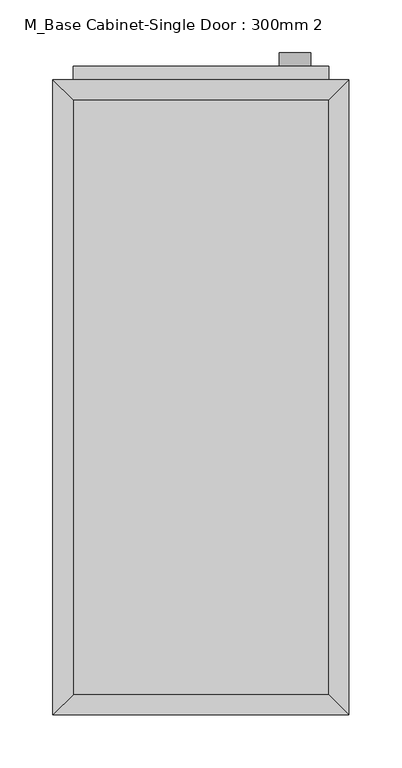
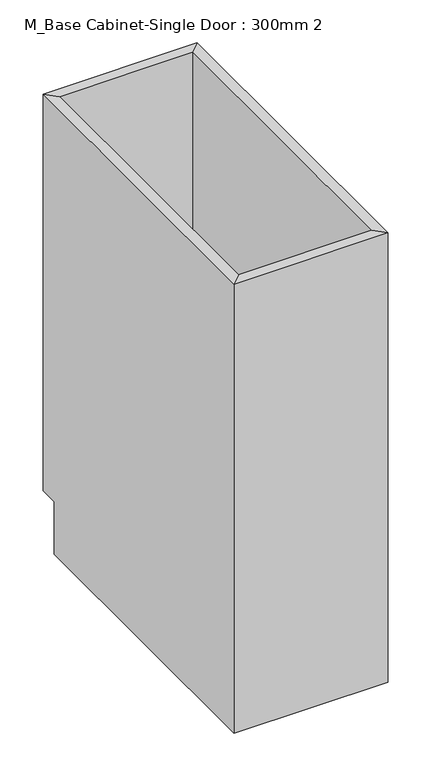
"""IFC4 building model written with IfcOpenShell, lengths in millimetres: furniture geometry, M_Base Cabinet-Single Door : 300mm 2."""

from ifc_helpers import new_model, si_unit, point, frame, frame_2d, origin, place, context, project, spatial, polyline, circle_curve, trimmed, segment, composite_curve, outline, extrude, faceted_brep, source, transform, mapped, element, save


def m_base_cabinet_single_door_300mm_2_2f133583(model_context):
    return source(origin(), model_context, "Body", "SolidModel", [
        faceted_brep([(139.3877049, 580.95, 860.0), (-101.9122951, 580.95, 860.0), (-101.9122951, 580.95, 100.0), (139.3877049, 580.95, 100.0), (158.4377049, 600.0, 860.0), (-120.9622951, 600.0, 860.0), (158.4377049, 600.0, 100.0), (-120.9622951, 600.0, 100.0), (-101.9122951, 19.05, 860.0), (-101.9122951, 19.05, 100.0), (-101.9122951, 565.0, 100.0), (-120.9622951, 0.0, 860.0), (-120.9622951, 565.0, 100.0), (-120.9622951, 565.0, 0.0), (-120.9622951, 0.0, 0.0), (139.3877049, 19.05, 860.0), (139.3877049, 19.05, 100.0), (158.4377049, 0.0, 860.0), (158.4377049, 0.0, 0.0), (139.3877049, 565.0, 100.0), (158.4377049, 565.0, 0.0), (158.4377049, 565.0, 100.0)], [[[0, 1, 2, 3]], [[0, 4, 5, 1]], [[4, 6, 7, 5]], [[2, 7, 6, 3]], [[1, 8, 9, 10, 2]], [[5, 11, 8, 1]], [[7, 12, 13, 14, 11, 5]], [[2, 10, 12, 7]], [[8, 15, 16, 9]], [[11, 17, 15, 8]], [[14, 18, 17, 11]], [[3, 19, 16, 15, 0]], [[0, 15, 17, 4]], [[4, 17, 18, 20, 21, 6]], [[6, 21, 19, 3]], [[10, 9, 16, 19]], [[18, 14, 13, 20]], [[13, 12, 10, 19, 21, 20]]]),
        extrude(outline(composite_curve([segment(trimmed(circle_curve(frame_2d((752.05, 107.6377049)), 15.0), [point((752.05, 92.6377049))], [point((752.05, 122.6377049))], False, "CARTESIAN"), True, "CONTINUOUS"), segment(trimmed(circle_curve(frame_2d((752.05, 107.6377049)), 15.0), [point((752.05, 122.6377049))], [point((752.05, 92.6377049))], False, "CARTESIAN"), True, "CONTINUOUS")], self_intersect=False)), frame((0.0, 612.7, 0.0), z_axis=(0.0, 1.0, 0.0), x_axis=(0.0, 0.0, 1.0)), (0.0, 0.0, 1.0), 12.7),
        extrude(outline(polyline([(139.3877049, 612.7), (139.3877049, 600.0), (-101.9122951, 600.0), (-101.9122951, 612.7), (139.3877049, 612.7)])), frame((0.0, 0.0, 119.05), z_axis=(0.0, 0.0, 1.0), x_axis=(1.0, 0.0, 0.0)), (0.0, 0.0, 1.0), 721.9),
        extrude(outline(polyline([(139.3877049, 19.05), (-101.9122951, 19.05), (-101.9122951, 580.95), (139.3877049, 580.95), (139.3877049, 19.05)])), frame((0.0, 0.0, 100.0), z_axis=(0.0, 0.0, 1.0), x_axis=(1.0, 0.0, 0.0)), (0.0, 0.0, 1.0), 19.05),
    ])


if __name__ == "__main__":
    model = new_model("IFC4")
    model_context = context("Model", 3, world=origin())
    ifc_project = project(units=[si_unit("LENGTHUNIT", "METRE", prefix="MILLI")], contexts=[model_context])
    site = spatial("IfcSite", under=ifc_project)
    building = spatial("IfcBuilding", under=site)
    placement = place(None, origin())
    m_base_cabinet_single_door_300mm_2_shape = m_base_cabinet_single_door_300mm_2_2f133583(model_context)
    element("IfcFurniture", 1, ObjectType="M_Base Cabinet-Single Door : 300mm 2", at=placement, inside=building, context=model_context, shape_type="MappedRepresentation", body=[
        mapped(m_base_cabinet_single_door_300mm_2_shape, transform((0.0, 0.0, 0.0), x_axis=(1.0, 0.0, 0.0), y_axis=(0.0, 1.0, 0.0), z_axis=(0.0, 0.0, 1.0))),
    ])
    save(model, "model.ifc")

# Revit data of these elements
# Type "M_Base Cabinet-Single Door : 300mm 2"
#   Depth = 1' - 11.62205"
#   Height = 2' - 9.85827"
#   Plinth Depth = 0' - 1.37795"
#   Plinth Height = 0' - 3.93701"
#   Width = 0' - 11"
#   Cabinet Material = Base cabinet 2120100 Aspekt - 83012120100 - White
#   Drawer Material = Base cabinet 2120100 Aspekt - 83012120100 - White
#   Handle Material = Cabinets - Handles
#   Default Elevation = 0
# Element 1 (IfcFurniture, "M_Base Cabinet-Single Door : 300mm 2")
#   Materials on its faces: "Base cabinet 2120100 Aspekt - 83012120100 - White", "Cabinets", "Cabinets - Handles"
# Materials
#   "Base cabinet 2120100 Aspekt - 83012120100 - White": class "Miscellaneous", colour RGB 255 255 255, transparency 0, Manufacturer = "Marbodal", URL = "http://www.marbodal.se", Cost = 0
#   "Cabinets - Handles": class "Metal", colour RGB 57 57 57, transparency 0
#   "Cabinets": class "Miscellaneous", colour RGB 249 249 249, transparency 0
